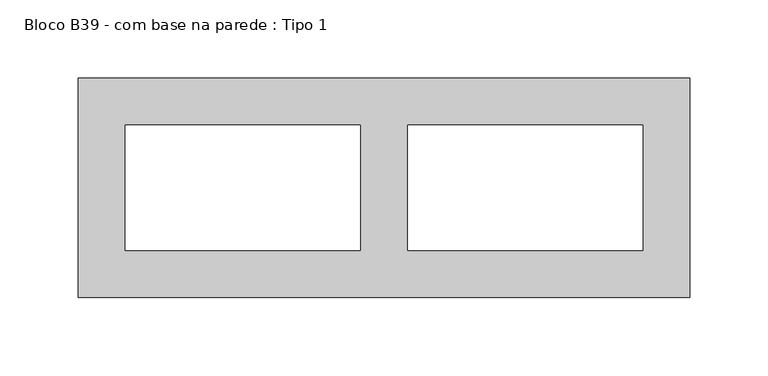
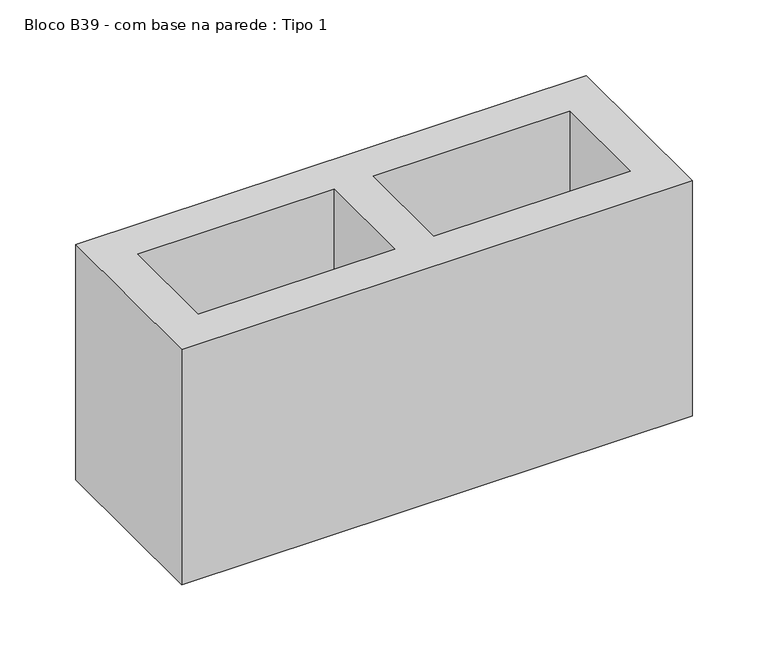
"""IFC4 building model written with IfcOpenShell, lengths in millimetres: proxy geometry, Bloco B39 - com base na parede : Tipo 1."""

from ifc_helpers import new_model, si_unit, origin, origin_with_axes, place, context, project, spatial, polyline, outline, extrude, source, transform, mapped, element, save


def bloco_b39_com_base_na_parede_tipo_1_b573ce29(model_context):
    return source(origin(), model_context, "Body", "SweptSolid", [
        extrude(outline(polyline([(320.0, 70.0), (320.0, -70.0), (-70.0, -70.0), (-70.0, 70.0), (320.0, 70.0)]), holes=[polyline([(110.0, 40.0), (-40.0, 40.0), (-40.0, -40.0), (110.0, -40.0), (110.0, 40.0)]), polyline([(140.0, 40.0), (140.0, -40.0), (290.0, -40.0), (290.0, 40.0), (140.0, 40.0)])]), origin_with_axes(), (0.0, 0.0, 1.0), 190.0),
    ])


if __name__ == "__main__":
    model = new_model("IFC4")
    model_context = context("Model", 3, world=origin())
    ifc_project = project(units=[si_unit("LENGTHUNIT", "METRE", prefix="MILLI")], contexts=[model_context])
    site = spatial("IfcSite", under=ifc_project)
    building = spatial("IfcBuilding", under=site)
    placement = place(None, origin())
    bloco_b39_com_base_na_parede_tipo_1_shape = bloco_b39_com_base_na_parede_tipo_1_b573ce29(model_context)
    element("IfcBuildingElementProxy", 1, Name="Bloco B39 - com base na parede : Tipo 1", ObjectType="Bloco B39 - com base na parede : Tipo 1", at=placement, inside=building, context=model_context, shape_type="MappedRepresentation", body=[
        mapped(bloco_b39_com_base_na_parede_tipo_1_shape, transform((0.0, 0.0, 0.0), x_axis=(1.0, 0.0, 0.0), y_axis=(0.0, 1.0, 0.0), z_axis=(0.0, 0.0, 1.0))),
    ])
    save(model, "model.ifc")

# Revit data of these elements
# Type "Bloco B39 - com base na parede : Tipo 1"
#   SINAPI = ""
#   Assembly Code = ""
